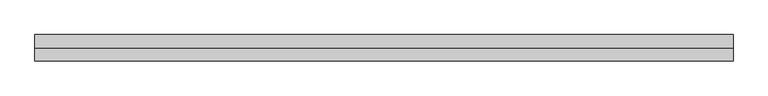
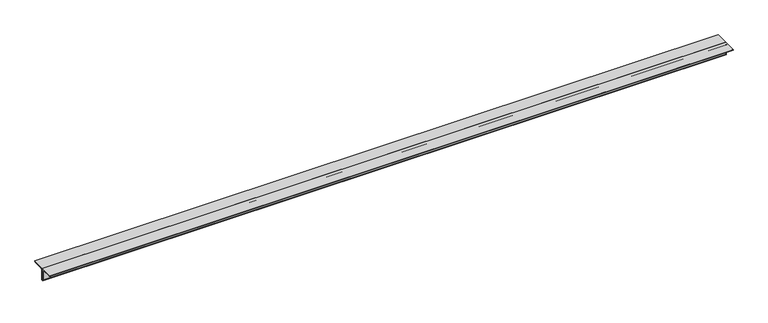
"""IFC4 building model written with IfcOpenShell, lengths in millimetres: member geometry, Steel Framing_2Ls_KS : H_SB_AR_S02_2Ls-100x100x10_VBR1."""

from ifc_helpers import new_model, si_unit, point, frame, frame_2d, origin, place, context, project, spatial, polyline, circle_curve, trimmed, segment, composite_curve, outline, extrude, source, transform, mapped, element, save


def member_5e8d3bf0(model_context):
    return source(origin(), model_context, "Body", "SweptSolid", [
        extrude(outline(composite_curve([segment(polyline([(0.0, 28.2), (100.0, 28.2)]), True, "CONTINUOUS"), segment(trimmed(circle_curve(frame_2d((90.0, 28.2)), 10.0), [point((100.0, 28.2))], [point((90.0, 18.2))], False, "CARTESIAN"), True, "CONTINUOUS"), segment(polyline([(90.0, 18.2), (20.0, 18.2)]), True, "CONTINUOUS"), segment(trimmed(circle_curve(frame_2d((20.0, 8.2)), 10.0), [point((20.0, 18.2))], [point((10.0, 8.2))], True, "CARTESIAN"), True, "CONTINUOUS"), segment(polyline([(10.0, 8.2), (10.0, -61.8)]), True, "CONTINUOUS"), segment(trimmed(circle_curve(frame_2d((0.0, -61.8)), 10.0), [point((10.0, -61.8))], [point((0.0, -71.8))], False, "CARTESIAN"), True, "CONTINUOUS"), segment(polyline([(0.0, -71.8), (0.0, 28.2)]), True, "CONTINUOUS")], self_intersect=False)), frame((-2444.561686, 0.0, 0.0), z_axis=(1.0, 0.0, 0.0), x_axis=(0.0, 1.0, 0.0)), (0.0, 0.0, 1.0), 5283.025664),
        extrude(outline(composite_curve([segment(polyline([(0.0, 28.2), (0.0, -71.8)]), True, "CONTINUOUS"), segment(trimmed(circle_curve(frame_2d((0.0, -61.8)), 10.0), [point((0.0, -71.8))], [point((-10.0, -61.8))], False, "CARTESIAN"), True, "CONTINUOUS"), segment(polyline([(-10.0, -61.8), (-10.0, 8.2)]), True, "CONTINUOUS"), segment(trimmed(circle_curve(frame_2d((-20.0, 8.2)), 10.0), [point((-10.0, 8.2))], [point((-20.0, 18.2))], True, "CARTESIAN"), True, "CONTINUOUS"), segment(polyline([(-20.0, 18.2), (-90.0, 18.2)]), True, "CONTINUOUS"), segment(trimmed(circle_curve(frame_2d((-90.0, 28.2)), 10.0), [point((-90.0, 18.2))], [point((-100.0, 28.2))], False, "CARTESIAN"), True, "CONTINUOUS"), segment(polyline([(-100.0, 28.2), (0.0, 28.2)]), True, "CONTINUOUS")], self_intersect=False)), frame((-2444.561686, 0.0, 0.0), z_axis=(1.0, 0.0, 0.0), x_axis=(0.0, 1.0, 0.0)), (0.0, 0.0, 1.0), 5283.025664),
    ])


if __name__ == "__main__":
    model = new_model("IFC4")
    model_context = context("Model", 3, world=origin())
    ifc_project = project(units=[si_unit("LENGTHUNIT", "METRE", prefix="MILLI")], contexts=[model_context])
    site = spatial("IfcSite", under=ifc_project)
    building = spatial("IfcBuilding", under=site)
    placement = place(None, origin())
    member_shape = member_5e8d3bf0(model_context)
    element("IfcMember", 1, ObjectType="Steel Framing_2Ls_KS : H_SB_AR_S02_2Ls-100x100x10_VBR1", at=placement, inside=building, context=model_context, shape_type="MappedRepresentation", body=[
        mapped(member_shape, transform((0.0, 0.0, 0.0), x_axis=(1.0, 0.0, 0.0), y_axis=(0.0, 1.0, 0.0), z_axis=(0.0, 0.0, 1.0))),
    ])
    save(model, "model.ifc")

# Revit data of these elements
# Type "Steel Framing_2Ls_KS : H_SB_AR_S02_2Ls-100x100x10_VBR1"
#   Type Comments = "MAIN"
#   Type Mark = "VBR1"
#   H_SectionID = "2Ls-100x100x10"
#   Assembly Code = "B10"
#   Legs = "LLBB"
#   H_Ratio for Additional Steel Plate = 0.2
#   W = 0
#   Perimeter = 0.80 m²/m
#   Nominal Weight = 29.80 kgf/m
#   Length [instance default] = 1524 mm
#   Space = 0 mm
#   b = 100 mm
#   d = 100 mm
#   t = 10 mm
#   y = 28.2 mm
#   A = 0.0038 m²
#   Structural Material [instance default] = Steel, 45-345
# Element 1 (IfcMember, "Steel Framing_2Ls_KS : H_SB_AR_S02_2Ls-100x100x10_VBR1")
#   Materials on its faces: "Steel, 45-345"
# Materials
#   "Steel, 45-345": class "Metal", colour RGB 189 187 185, transparency 0, Description = "Steel 345 MPa", Cost = 0
